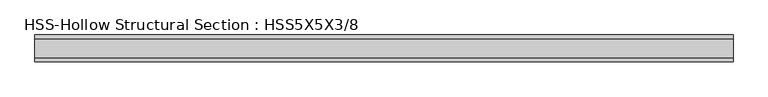
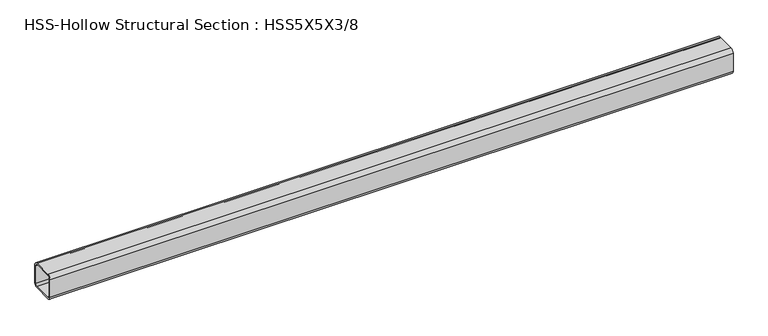
"""IFC4 building model written with IfcOpenShell, lengths in millimetres: member geometry, HSS-Hollow Structural Section : HSS5X5X3/8."""

import ifcopenshell
import ifcopenshell.guid

model = None  # the IFC model being written
_history = None  # IfcOwnerHistory: only IFC2X3 demands one
_inside = {}  # id of a spatial element -> (the spatial element, [elements in it])
_under = {}  # id of a project, library or spatial element -> (it, [spatial elements below it])
_declared = {}  # id of a project -> (the project, [libraries it declares])
_typed = {}  # id of a type object -> (the type object, [elements of that type])
_made_of = {}  # id of a material, layer set ... -> (it, [elements and type objects made of it])


def new_model(schema):
    """Start an empty IFC model of exactly this schema.

    Asked for "IFC4X3", IfcOpenShell would pick the latest addendum, in which some entities
    have other attributes; the version numbers below select the first issue.
    IFC2X3 requires an IfcOwnerHistory on every rooted entity: one is made here for all.
    """
    global model, _history
    if schema == "IFC4X3":
        model = ifcopenshell.file(schema_version=(4, 3, 0, 0))
    else:
        model = ifcopenshell.file(schema=schema)
    _inside.clear()
    _under.clear()
    _declared.clear()
    _typed.clear()
    _made_of.clear()
    _history = None
    if model.schema == "IFC2X3":
        org = make("IfcOrganization", Name="unknown")
        user = make(
            "IfcPersonAndOrganization",
            ThePerson=make("IfcPerson", FamilyName="unknown"),
            TheOrganization=org,
        )
        app = make(
            "IfcApplication",
            ApplicationDeveloper=org,
            Version="unknown",
            ApplicationFullName="unknown",
            ApplicationIdentifier="unknown",
        )
        _history = make(
            "IfcOwnerHistory",
            OwningUser=user,
            OwningApplication=app,
            ChangeAction="ADDED",
            CreationDate=0,
        )
    return model


def make(cls, **values):
    """One entity of the class cls with the attributes given. An attribute that is None is left unset."""
    return model.create_entity(
        cls, **{name: value for name, value in values.items() if value is not None}
    )


def rooted(cls, **values):
    """An entity with a GlobalId (a new one), such as an element, a storey or a relation."""
    return make(cls, GlobalId=ifcopenshell.guid.new(), OwnerHistory=_history, **values)


def si_unit(unit_type, name, prefix=None):
    """IfcSIUnit, for example si_unit("LENGTHUNIT", "METRE", prefix="MILLI")."""
    return make("IfcSIUnit", UnitType=unit_type, Prefix=prefix, Name=name)


def assignment(units):
    """IfcUnitAssignment: the units of a project."""
    return None if units is None else make("IfcUnitAssignment", Units=units)


def point(xyz):
    """IfcCartesianPoint."""
    return None if xyz is None else make("IfcCartesianPoint", Coordinates=xyz)


def direction(xyz):
    """IfcDirection."""
    return None if xyz is None else make("IfcDirection", DirectionRatios=xyz)


def frame(location, z_axis=None, x_axis=None):
    """IfcAxis2Placement3D, a coordinate frame: its origin and axes. An axis left out is left unset."""
    return make(
        "IfcAxis2Placement3D",
        Location=point(location),
        Axis=direction(z_axis),
        RefDirection=direction(x_axis),
    )


def frame_2d(location, x_axis=None):
    """IfcAxis2Placement2D, a coordinate frame in the plane: its origin and x axis."""
    return make(
        "IfcAxis2Placement2D", Location=point(location), RefDirection=direction(x_axis)
    )


def origin():
    """The frame at (0, 0, 0) with its axes left unset."""
    return frame((0.0, 0.0, 0.0))


def place(relative_to, where):
    """IfcLocalPlacement: puts the frame where relative to a parent placement (None: the world)."""
    return make(
        "IfcLocalPlacement", PlacementRelTo=relative_to, RelativePlacement=where
    )


def context(
    kind, dimensions, precision=None, world=None, true_north=None, identifier=None
):
    """IfcGeometricRepresentationContext, for example the 3D "Model" context."""
    return make(
        "IfcGeometricRepresentationContext",
        ContextIdentifier=identifier,
        ContextType=kind,
        CoordinateSpaceDimension=dimensions,
        Precision=precision,
        WorldCoordinateSystem=world,
        TrueNorth=true_north,
    )


def project(units=None, contexts=None):
    """IfcProject with its units and contexts."""
    return rooted(
        "IfcProject",
        Name="project",
        RepresentationContexts=contexts,
        UnitsInContext=assignment(units),
    )


def spatial(cls, under=None, at=None, **own):
    """A site, building, storey or space (cls), placed at a placement, below another one or the project."""
    s = rooted(cls, ObjectPlacement=at, **own)
    if under is not None:
        _under.setdefault(under.id(), (under, []))[1].append(s)
    return s


def polyline(points):
    """IfcPolyline through the points."""
    return make("IfcPolyline", Points=[point(p) for p in points])


def circle_curve(where, radius):
    """IfcCircle in the frame where."""
    return make("IfcCircle", Position=where, Radius=radius)


def trimmed(basis, trim1, trim2, sense, master):
    """IfcTrimmedCurve: the piece of a basis curve between two trims."""
    return make(
        "IfcTrimmedCurve",
        BasisCurve=basis,
        Trim1=trim1,
        Trim2=trim2,
        SenseAgreement=sense,
        MasterRepresentation=master,
    )


def segment(curve, same_sense, transition):
    """IfcCompositeCurveSegment."""
    return make(
        "IfcCompositeCurveSegment",
        Transition=transition,
        SameSense=same_sense,
        ParentCurve=curve,
    )


def composite_curve(segments, self_intersect=None):
    """IfcCompositeCurve: segments joined end to end."""
    return make("IfcCompositeCurve", Segments=segments, SelfIntersect=self_intersect)


def outline(outer, holes=None, kind="AREA"):
    """IfcArbitraryClosedProfileDef: a profile drawn as a closed curve; with holes, ...WithVoids."""
    if holes is None:
        return make("IfcArbitraryClosedProfileDef", ProfileType=kind, OuterCurve=outer)
    return make(
        "IfcArbitraryProfileDefWithVoids",
        ProfileType=kind,
        OuterCurve=outer,
        InnerCurves=holes,
    )


def extrude(swept, where, along, depth):
    """IfcExtrudedAreaSolid: the profile swept, set in the frame where, extruded along a direction by depth."""
    return make(
        "IfcExtrudedAreaSolid",
        SweptArea=swept,
        Position=where,
        ExtrudedDirection=direction(along),
        Depth=depth,
    )


def shape(context_of_items, identifier, shape_type, items):
    """IfcShapeRepresentation: the items that make up one representation, for example the "Body"."""
    return make(
        "IfcShapeRepresentation",
        ContextOfItems=context_of_items,
        RepresentationIdentifier=identifier,
        RepresentationType=shape_type,
        Items=items,
    )


def source(mapping_origin, context_of_items, identifier, shape_type, items):
    """IfcRepresentationMap: a shape defined once, which mapped items show again and again."""
    return make(
        "IfcRepresentationMap",
        MappingOrigin=mapping_origin,
        MappedRepresentation=shape(context_of_items, identifier, shape_type, items),
    )


def transform(
    local_origin,
    x_axis=None,
    y_axis=None,
    z_axis=None,
    scale=None,
    scale2=None,
    scale3=None,
    uniform=True,
):
    """IfcCartesianTransformationOperator3D, or its non-uniform kind. x_axis, y_axis, z_axis: its Axis1, 2, 3."""
    if uniform:
        return make(
            "IfcCartesianTransformationOperator3D",
            Axis1=direction(x_axis),
            Axis2=direction(y_axis),
            LocalOrigin=point(local_origin),
            Scale=scale,
            Axis3=direction(z_axis),
        )
    return make(
        "IfcCartesianTransformationOperator3DnonUniform",
        Axis1=direction(x_axis),
        Axis2=direction(y_axis),
        LocalOrigin=point(local_origin),
        Scale=scale,
        Axis3=direction(z_axis),
        Scale2=scale2,
        Scale3=scale3,
    )


def mapped(mapping_source, mapping_target):
    """IfcMappedItem: shows the shape of a source again, moved by a transform."""
    return make(
        "IfcMappedItem", MappingSource=mapping_source, MappingTarget=mapping_target
    )


def made_of(thing, what):
    """Note that an element or type object is made of a material, layer set ...; save() writes the relation."""
    if what is not None:
        _made_of.setdefault(what.id(), (what, []))[1].append(thing)
    return thing


def element(
    cls,
    number,
    at=None,
    inside=None,
    cuts=None,
    type_object=None,
    material=None,
    context=None,
    identifier="Body",
    shape_type=None,
    held_by="IfcProductDefinitionShape",
    body=None,
    shapes=None,
    **own,
):
    """One element of the class cls, such as IfcWall. Its Tag is "e" and its number.

    at: its placement. inside: the storey or other place that contains it. cuts: it is an
    opening in that element (IfcRelVoidsElement). A single representation is given by context,
    identifier, shape_type and body (its items); several are given by shapes. held_by: the class
    of the entity that holds the representations. save() writes the other relations.
    """
    e = rooted(cls, Tag="e%d" % number, ObjectPlacement=at, **own)
    if body is not None:
        shapes = [shape(context, identifier, shape_type, body)]
    if shapes is not None:
        e.Representation = make(held_by, Representations=shapes)
    if inside is not None:
        _inside.setdefault(inside.id(), (inside, []))[1].append(e)
    if cuts is not None:
        rooted(
            "IfcRelVoidsElement", RelatingBuildingElement=cuts, RelatedOpeningElement=e
        )
    if type_object is not None:
        _typed.setdefault(type_object.id(), (type_object, []))[1].append(e)
    return made_of(e, material)


def aggregate(whole, parts):
    """IfcRelAggregates: a whole, such as a stair, and the parts it consists of."""
    return rooted("IfcRelAggregates", RelatingObject=whole, RelatedObjects=parts)


def save(model, path):
    """Write the relations noted so far, then the file.

    IfcRelAggregates (storeys below a building ...), IfcRelContainedInSpatialStructure (elements
    in a storey), IfcRelDefinesByType, IfcRelAssociatesMaterial and IfcRelDeclares: one each for
    every whole, place, type object, material and project.
    """
    for whole, parts in _under.values():
        aggregate(whole, parts)
    for where, things in _inside.values():
        rooted(
            "IfcRelContainedInSpatialStructure",
            RelatedElements=things,
            RelatingStructure=where,
        )
    for kind, things in _typed.values():
        rooted("IfcRelDefinesByType", RelatedObjects=things, RelatingType=kind)
    for what, things in _made_of.values():
        rooted("IfcRelAssociatesMaterial", RelatedObjects=things, RelatingMaterial=what)
    for by, libraries in _declared.values():
        rooted("IfcRelDeclares", RelatingContext=by, RelatedDefinitions=libraries)
    model.write(path)


def hss_hollow_structural_section_hss5x5x3_8_017cef90(model_context):
    return source(origin(), model_context, "Body", "SweptSolid", [
        extrude(outline(composite_curve([segment(polyline([(63.5, 45.7708), (63.5, -45.7708)]), True, "CONTINUOUS"), segment(trimmed(circle_curve(frame_2d((45.7708, -45.7708)), 17.7292), [point((63.5, -45.7708))], [point((45.7708, -63.5))], False, "CARTESIAN"), True, "CONTINUOUS"), segment(polyline([(45.7708, -63.5), (-45.7708, -63.5)]), True, "CONTINUOUS"), segment(trimmed(circle_curve(frame_2d((-45.7708, -45.7708)), 17.7292), [point((-45.7708, -63.5))], [point((-63.5, -45.7708))], False, "CARTESIAN"), True, "CONTINUOUS"), segment(polyline([(-63.5, -45.7708), (-63.5, 45.7708)]), True, "CONTINUOUS"), segment(trimmed(circle_curve(frame_2d((-45.7708, 45.7708)), 17.7292), [point((-63.5, 45.7708))], [point((-45.7708, 63.5))], False, "CARTESIAN"), True, "CONTINUOUS"), segment(polyline([(-45.7708, 63.5), (45.7708, 63.5)]), True, "CONTINUOUS"), segment(trimmed(circle_curve(frame_2d((45.7708, 45.7708)), 17.7292), [point((45.7708, 63.5))], [point((63.5, 45.7708))], False, "CARTESIAN"), True, "CONTINUOUS")], self_intersect=False), holes=[composite_curve([segment(trimmed(circle_curve(frame_2d((-45.7708, 45.7708)), 8.8646), [point((-45.7708, 54.6354))], [point((-54.6354, 45.7708))], True, "CARTESIAN"), True, "CONTINUOUS"), segment(polyline([(-54.6354, 45.7708), (-54.6354, -45.7708)]), True, "CONTINUOUS"), segment(trimmed(circle_curve(frame_2d((-45.7708, -45.7708)), 8.8646), [point((-54.6354, -45.7708))], [point((-45.7708, -54.6354))], True, "CARTESIAN"), True, "CONTINUOUS"), segment(polyline([(-45.7708, -54.6354), (45.7708, -54.6354)]), True, "CONTINUOUS"), segment(trimmed(circle_curve(frame_2d((45.7708, -45.7708)), 8.8646), [point((45.7708, -54.6354))], [point((54.6354, -45.7708))], True, "CARTESIAN"), True, "CONTINUOUS"), segment(polyline([(54.6354, -45.7708), (54.6354, 45.7708)]), True, "CONTINUOUS"), segment(trimmed(circle_curve(frame_2d((45.7708, 45.7708)), 8.8646), [point((54.6354, 45.7708))], [point((45.7708, 54.6354))], True, "CARTESIAN"), True, "CONTINUOUS"), segment(polyline([(45.7708, 54.6354), (-45.7708, 54.6354)]), True, "CONTINUOUS")], self_intersect=False)]), frame((-1660.5512918, 0.0, 0.0), z_axis=(1.0, 0.0, 0.0), x_axis=(0.0, 1.0, 0.0)), (0.0, 0.0, 1.0), 3321.1025836),
    ])


if __name__ == "__main__":
    model = new_model("IFC4")
    model_context = context("Model", 3, world=origin())
    ifc_project = project(units=[si_unit("LENGTHUNIT", "METRE", prefix="MILLI")], contexts=[model_context])
    site = spatial("IfcSite", under=ifc_project)
    building = spatial("IfcBuilding", under=site)
    placement = place(None, origin())
    hss_hollow_structural_section_hss5x5x3_8_shape = hss_hollow_structural_section_hss5x5x3_8_017cef90(model_context)
    element("IfcMember", 1, ObjectType="HSS-Hollow Structural Section : HSS5X5X3/8", at=placement, inside=building, context=model_context, shape_type="MappedRepresentation", body=[
        mapped(hss_hollow_structural_section_hss5x5x3_8_shape, transform((0.0, 0.0, 0.0), x_axis=(1.0, 0.0, 0.0), y_axis=(0.0, 1.0, 0.0), z_axis=(0.0, 0.0, 1.0))),
    ])
    save(model, "model.ifc")

# Revit data of these elements
# Type "HSS-Hollow Structural Section : HSS5X5X3/8"
#   Assembly Code = "B10"
#   Shape = "Square"
#   W = 22.3
#   Ht = 0' - 5"
#   Length [instance default] = 5' - 0"
#   b = 0' - 5"
#   kr = 0' - 0.698"
#   t = 0' - 0.349"
#   A = 0.0429167 SF
#   Structural Material [instance default] = Steel ASTM A500, Grade B, Rectangular and Square
# Element 1 (IfcMember, "HSS-Hollow Structural Section : HSS5X5X3/8")
#   Materials on its faces: "Steel ASTM A500, Grade B, Rectangular and Square"
# Materials
#   "Steel ASTM A500, Grade B, Rectangular and Square": class "Metal", colour RGB 199 199 199, transparency 0, Description = "Carbon steel", Cost = 0
